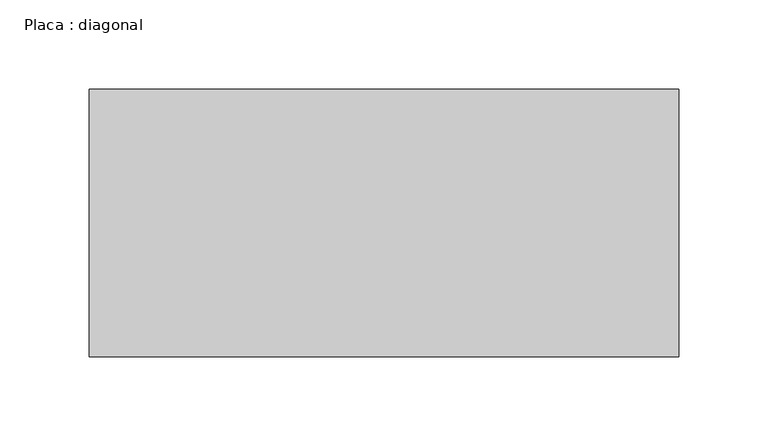
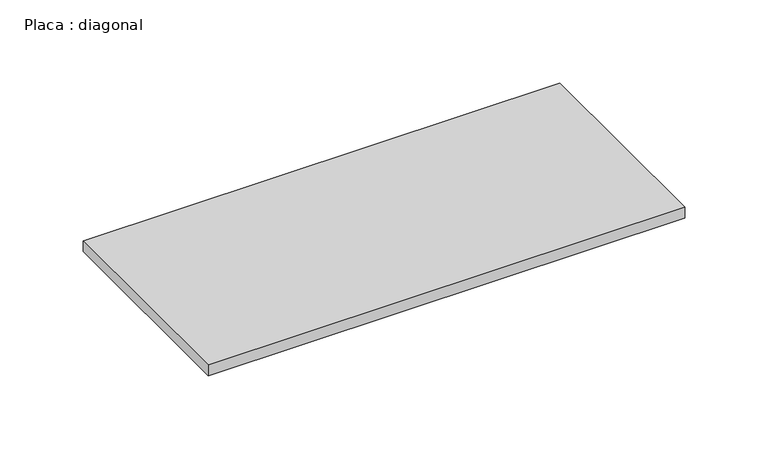
"""IFC4 building model written with IfcOpenShell, lengths in millimetres: beam geometry, Placa : diagonal."""

from ifc_helpers import new_model, si_unit, frame, origin, place, context, project, spatial, polyline, outline, extrude, source, transform, mapped, element, save


def placa_diagonal_5ef1143b(model_context):
    return source(origin(), model_context, "Body", "SweptSolid", [
        extrude(outline(polyline([(165.496273, 75.0), (165.496273, -75.0), (-165.1705217, -75.0), (-165.1705217, 75.0), (165.496273, 75.0)])), frame((0.0, 0.0, -4.0), z_axis=(0.0, 0.0, 1.0), x_axis=(1.0, 0.0, 0.0)), (0.0, 0.0, 1.0), 8.0),
    ])


if __name__ == "__main__":
    model = new_model("IFC4")
    model_context = context("Model", 3, world=origin())
    ifc_project = project(units=[si_unit("LENGTHUNIT", "METRE", prefix="MILLI")], contexts=[model_context])
    site = spatial("IfcSite", under=ifc_project)
    building = spatial("IfcBuilding", under=site)
    placement = place(None, origin())
    placa_diagonal_shape = placa_diagonal_5ef1143b(model_context)
    element("IfcBeam", 1, ObjectType="Placa : diagonal", at=placement, inside=building, context=model_context, shape_type="MappedRepresentation", body=[
        mapped(placa_diagonal_shape, transform((0.0, 0.0, 0.0), x_axis=(1.0, 0.0, 0.0), y_axis=(0.0, 1.0, 0.0), z_axis=(0.0, 0.0, 1.0))),
    ])
    save(model, "model.ifc")

# Revit data of these elements
# Type "Placa : diagonal"
#   W = 0
#   Length [instance default] = 1.50 m
#   b = 0.15 m
#   d = 0.008 m
#   A = 0 m²
#   Structural Material [instance default] = Aço, 45-345
# Element 1 (IfcBeam, "Placa : diagonal")
#   Materials on its faces: "Aço, 45-345"
# Materials
#   "Aço, 45-345": class "Metal", colour RGB 247 247 247, transparency 0, Description = "Aço 345 MPa", Cost = 0
